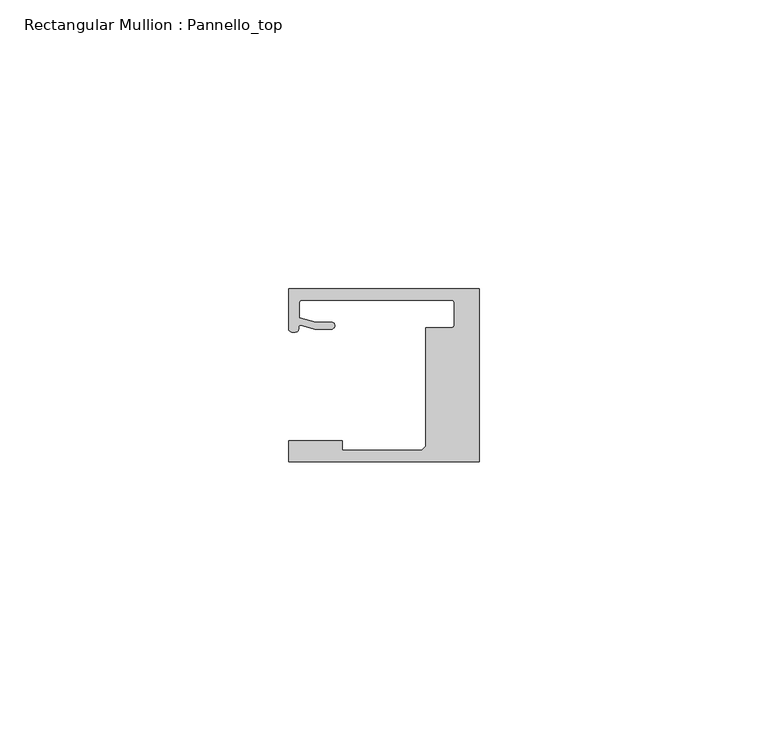
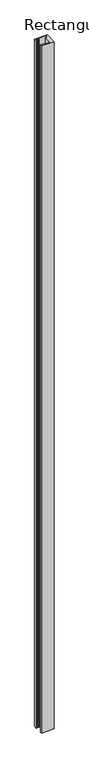
"""IFC4 building model written with IfcOpenShell, lengths in millimetres: member geometry, Rectangular Mullion : Pannello_top."""

from ifc_helpers import new_model, si_unit, frame, origin, place, context, project, spatial, polyline, circle_curve, source, transform, mapped, element, save
from ifc_brep_helpers import plane_surface, cylinder_surface, revolved_surface, extruded_surface, spline_curve, advanced_brep


def rectangular_mullion_pannello_top_e9d0786e(model_context):
    return source(origin(), model_context, "Body", "AdvancedBrep", [
        advanced_brep(
        [(-33.0, -15.0, 0.0), (0.0, -15.0, 0.0), (0.0, 15.0, 0.0), (-33.0000135, 15.0, 0.0), (-33.0000135, 8.0000472, 0.0), (-30.9223017, 8.6490241, 0.0), (-28.4999305, 7.9999523, 0.0), (-25.59998, 7.9999523, 0.0), (-25.59998, 9.1999523, 0.0), (-28.3419477, 9.1999523, 0.0), (-31.19998, 9.9657591, 0.0), (-31.19998, 12.50001, 0.0), (-30.69998, 13.00001, 0.0), (-4.7999726, 13.00001, 0.0), (-4.2999726, 12.50001, 0.0), (-4.2999726, 8.7500595, 0.0), (-4.7999726, 8.2500595, 0.0), (-9.2999726, 8.2500595, 0.0), (-9.2999726, -12.2999849, 0.0), (-10.0000103, -13.0000004, 0.0), (-23.700041, -13.0000004, 0.0), (-23.700041, -11.3000004, 0.0), (-33.0, -11.3000004, 0.0), (-33.0, -15.0, -1883.9999729), (-33.0, -11.3000004, -1883.9999729), (-23.700041, -11.3000004, -1883.9999729), (-23.700041, -13.0000004, -1883.9999729), (-10.0000103, -13.0000004, -1883.9999729), (-9.2999726, -12.2999849, -1883.9999729), (-9.2999726, 8.2500595, -1883.9999729), (-4.7999726, 8.2500595, -1883.9999729), (-4.2999726, 8.7500595, -1883.9999729), (-4.2999726, 12.50001, -1883.9999729), (-4.7999726, 13.00001, -1883.9999729), (-30.69998, 13.00001, -1883.9999729), (-31.19998, 12.50001, -1883.9999729), (-31.19998, 9.9657591, -1883.9999729), (-28.3419477, 9.1999523, -1883.9999729), (-25.59998, 9.1999523, -1883.9999729), (-25.59998, 7.9999523, -1883.9999729), (-28.4999305, 7.9999523, -1883.9999729), (-30.9223017, 8.6490241, -1883.9999729), (-33.0000135, 8.0000472, -1883.9999729), (-33.0000135, 15.0, -1883.9999729), (0.0, 15.0, -1883.9999729), (0.0, -15.0, -1883.9999729)],
        [
            (0, 1),
            (1, 2),
            (2, 3),
            (3, 4),
            (4, 5, spline_curve(3, [(-33.0000135, 8.0000472, 0.0), (-33.0000135, 7.457047519, 0.0), (-32.262327879, 7.456527435, 0.0), (-31.357433266, 7.563996614, 0.0), (-31.305645054, 7.690065204, 0.0), (-31.298563602, 8.366228555, 0.0), (-31.312054066, 8.717747958, 0.0), (-30.9223017, 8.6490241, 0.0)], [4, 2, 2, 4], [0.0, 0.0027053965905959043, 0.0058611956533709, 0.007702013405570312])),
            (5, 6),
            (6, 7),
            (7, 8, circle_curve(frame((-25.59998, 8.5999523, 0.0), z_axis=(0.0, 0.0, 1.0), x_axis=(0.0, 1.0, 0.0)), 0.6)),
            (8, 9),
            (9, 10),
            (10, 11),
            (11, 12, circle_curve(frame((-30.69998, 12.50001, 0.0), z_axis=(0.0, 0.0, -1.0), x_axis=(0.0, 1.0, 0.0)), 0.5)),
            (12, 13),
            (13, 14, circle_curve(frame((-4.7999726, 12.50001, 0.0), z_axis=(0.0, 0.0, -1.0), x_axis=(1.0, 0.0, 0.0)), 0.5)),
            (14, 15),
            (15, 16, circle_curve(frame((-4.7999726, 8.7500595, 0.0), z_axis=(0.0, 0.0, -1.0), x_axis=(0.0, -1.0, 0.0)), 0.5)),
            (16, 17),
            (17, 18),
            (18, 19),
            (19, 20),
            (20, 21),
            (21, 22),
            (22, 0),
            (23, 24),
            (24, 25),
            (25, 26),
            (26, 27),
            (27, 28),
            (28, 29),
            (29, 30),
            (30, 31, circle_curve(frame((-4.7999726, 8.7500595, -1883.9999729), z_axis=(0.0, 0.0, 1.0), x_axis=(0.0, -1.0, 0.0)), 0.5)),
            (31, 32),
            (32, 33, circle_curve(frame((-4.7999726, 12.50001, -1883.9999729), z_axis=(0.0, 0.0, 1.0), x_axis=(1.0, 0.0, 0.0)), 0.5)),
            (33, 34),
            (34, 35, circle_curve(frame((-30.69998, 12.50001, -1883.9999729), z_axis=(0.0, 0.0, 1.0), x_axis=(0.0, 1.0, 0.0)), 0.5)),
            (35, 36),
            (36, 37),
            (37, 38),
            (38, 39, circle_curve(frame((-25.59998, 8.5999523, -1883.9999729), z_axis=(0.0, 0.0, -1.0), x_axis=(0.0, 1.0, 0.0)), 0.6)),
            (39, 40),
            (40, 41),
            (41, 42, spline_curve(3, [(-30.9223017, 8.6490241, -1883.9999729), (-31.312054066, 8.717747958, -1883.9999729), (-31.298563602, 8.366228555, -1883.9999729), (-31.305645054, 7.690065204, -1883.9999729), (-31.357433266, 7.563996614, -1883.9999729), (-32.262327879, 7.456527435, -1883.9999729), (-33.0000135, 7.457047519, -1883.9999729), (-33.0000135, 8.0000472, -1883.9999729)], [4, 2, 2, 4], [0.0, 0.001840817752199412, 0.004996616814974408, 0.007702013405570312])),
            (42, 43),
            (43, 44),
            (44, 45),
            (45, 23),
            (0, 23),
            (45, 1),
            (44, 2),
            (43, 3),
            (42, 4),
            (41, 5),
            (40, 6),
            (39, 7),
            (38, 8),
            (37, 9),
            (36, 10),
            (35, 11),
            (34, 12),
            (33, 13),
            (32, 14),
            (31, 15),
            (30, 16),
            (29, 17),
            (28, 18),
            (27, 19),
            (26, 20),
            (25, 21),
            (24, 22),
        ],
        [
            plane_surface(frame((0.0, -36.2491502, 0.0), z_axis=(0.0, 0.0, 1.0), x_axis=(-1.0, 0.0, 0.0))),
            plane_surface(frame((0.0, -36.2491502, -1883.9999729), z_axis=(0.0, 0.0, -1.0), x_axis=(-1.0, 0.0, 0.0))),
            plane_surface(frame((-33.0, -15.0, 0.0), z_axis=(0.0, -1.0, 0.0), x_axis=(0.0, 0.0, -1.0))),
            plane_surface(frame((0.0, -15.0, 0.0), z_axis=(1.0, 0.0, 0.0), x_axis=(0.0, 0.0, -1.0))),
            plane_surface(frame((0.0, 15.0, 0.0), z_axis=(0.0, 1.0, 0.0), x_axis=(0.0, 0.0, -1.0))),
            plane_surface(frame((-33.0000135, 15.0, 0.0), z_axis=(-1.0, 0.0, 0.0), x_axis=(0.0, 0.0, -1.0))),
            extruded_surface(spline_curve(3, [(-33.0000135, 8.0000472, -1883.9999729), (-33.0000135, 7.457047519, -1883.9999729), (-32.262327879, 7.456527435, -1883.9999729), (-31.357433266, 7.563996614, -1883.9999729), (-31.305645054, 7.690065204, -1883.9999729), (-31.298563602, 8.366228555, -1883.9999729), (-31.312054066, 8.717747958, -1883.9999729), (-30.9223017, 8.6490241, -1883.9999729)], [4, 2, 2, 4], [0.0, 0.0027053965905959043, 0.0058611956533709, 0.007702013405570312]), (0.0, 0.0, 1883.9999729), 1883.9999729),
            plane_surface(frame((-30.9223017, 8.6490241, 0.0), z_axis=(-0.25881883200192934, -0.9659258833891746, 0.0), x_axis=(0.0, 0.0, -1.0))),
            plane_surface(frame((-28.4999305, 7.9999523, 0.0), z_axis=(0.0, -1.0, 0.0), x_axis=(0.0, 0.0, -1.0))),
            cylinder_surface(frame((-25.59998, 8.5999523, 0.0), z_axis=(0.0, 0.0, 1.0), x_axis=(0.0, 1.0, 0.0)), 0.6),
            plane_surface(frame((-25.59998, 9.1999523, 0.0), z_axis=(0.0, 1.0, 0.0), x_axis=(0.0, 0.0, -1.0))),
            plane_surface(frame((-28.3419477, 9.1999523, 0.0), z_axis=(0.25881883204288636, 0.9659258833782002, 0.0), x_axis=(0.0, 0.0, -1.0))),
            plane_surface(frame((-31.19998, 9.9657591, 0.0), z_axis=(1.0, 0.0, 0.0), x_axis=(0.0, 0.0, -1.0))),
            revolved_surface(polyline([(-30.69998, 13.00001, -1883.9999729), (-30.69998, 13.00001, 0.0)]), (-30.69998, 12.50001, 0.0), (0.0, 0.0, -1.0)),
            plane_surface(frame((-30.69998, 13.00001, 0.0), z_axis=(0.0, -1.0, 0.0), x_axis=(0.0, 0.0, -1.0))),
            revolved_surface(polyline([(-4.2999726, 12.50001, -1883.9999729), (-4.2999726, 12.50001, 0.0)]), (-4.7999726, 12.50001, 0.0), (0.0, 0.0, -1.0)),
            plane_surface(frame((-4.2999726, 12.50001, 0.0), z_axis=(-1.0, 0.0, 0.0), x_axis=(0.0, 0.0, -1.0))),
            revolved_surface(polyline([(-4.7999726, 8.2500595, -1883.9999729), (-4.7999726, 8.2500595, 0.0)]), (-4.7999726, 8.7500595, 0.0), (0.0, 0.0, -1.0)),
            plane_surface(frame((-4.7999726, 8.2500595, 0.0), z_axis=(0.0, 1.0, 0.0), x_axis=(0.0, 0.0, -1.0))),
            plane_surface(frame((-9.2999726, 8.2500595, 0.0), z_axis=(-1.0, 0.0, 0.0), x_axis=(0.0, 0.0, -1.0))),
            plane_surface(frame((-9.2999726, -12.2999849, 0.0), z_axis=(-0.7070955486277984, 0.7071180135668678, 0.0), x_axis=(0.0, 0.0, -1.0))),
            plane_surface(frame((-10.0000103, -13.0000004, 0.0), z_axis=(0.0, 1.0, 0.0), x_axis=(0.0, 0.0, -1.0))),
            plane_surface(frame((-23.700041, -13.0000004, 0.0), z_axis=(1.0, 0.0, 0.0), x_axis=(0.0, 0.0, -1.0))),
            plane_surface(frame((-23.700041, -11.3000004, 0.0), z_axis=(0.0, 1.0, 0.0), x_axis=(0.0, 0.0, -1.0))),
            plane_surface(frame((-33.0, -11.3000004, 0.0), z_axis=(-1.0, 0.0, 0.0), x_axis=(0.0, 0.0, -1.0))),
        ],
        [
            (0, [[1, 2, 3, 4, 5, 6, 7, 8, 9, 10, 11, 12, 13, 14, 15, 16, 17, 18, 19, 20, 21, 22, 23]]),
            (1, [[24, 25, 26, 27, 28, 29, 30, 31, 32, 33, 34, 35, 36, 37, 38, 39, 40, 41, 42, 43, 44, 45, 46]]),
            (2, [[-1, 47, -46, 48]]),
            (3, [[-2, -48, -45, 49]]),
            (4, [[-3, -49, -44, 50]]),
            (5, [[-4, -50, -43, 51]]),
            (6, [[-5, -51, -42, 52]]),
            (7, [[-6, -52, -41, 53]]),
            (8, [[-7, -53, -40, 54]]),
            (9, [[-8, -54, -39, 55]]),
            (10, [[-9, -55, -38, 56]]),
            (11, [[-10, -56, -37, 57]]),
            (12, [[-11, -57, -36, 58]]),
            (13, [[-12, -58, -35, 59]]),
            (14, [[-13, -59, -34, 60]]),
            (15, [[-14, -60, -33, 61]]),
            (16, [[-15, -61, -32, 62]]),
            (17, [[-16, -62, -31, 63]]),
            (18, [[-17, -63, -30, 64]]),
            (19, [[-18, -64, -29, 65]]),
            (20, [[-19, -65, -28, 66]]),
            (21, [[-20, -66, -27, 67]]),
            (22, [[-21, -67, -26, 68]]),
            (23, [[-22, -68, -25, 69]]),
            (24, [[-23, -69, -24, -47]]),
        ],
    ),
    ])


if __name__ == "__main__":
    model = new_model("IFC4")
    model_context = context("Model", 3, world=origin())
    ifc_project = project(units=[si_unit("LENGTHUNIT", "METRE", prefix="MILLI")], contexts=[model_context])
    site = spatial("IfcSite", under=ifc_project)
    building = spatial("IfcBuilding", under=site)
    placement = place(None, origin())
    rectangular_mullion_pannello_top_shape = rectangular_mullion_pannello_top_e9d0786e(model_context)
    element("IfcMember", 1, ObjectType="Rectangular Mullion : Pannello_top", at=placement, inside=building, context=model_context, shape_type="MappedRepresentation", body=[
        mapped(rectangular_mullion_pannello_top_shape, transform((0.0, 0.0, 0.0), x_axis=(1.0, 0.0, 0.0), y_axis=(0.0, 1.0, 0.0), z_axis=(0.0, 0.0, 1.0))),
    ])
    save(model, "model.ifc")

# Revit data of these elements
# Type "Rectangular Mullion : Pannello_top"
#   built-in parameter 1007322 = 0.0984252 (stored number, unit not read)
#   built-in parameter 1007321 = 0 (stored number, unit not read)
#   built-in parameter 1007320 = 0.0305117 (stored number, unit not read)
